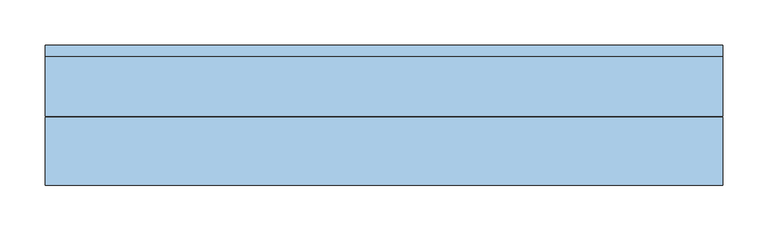
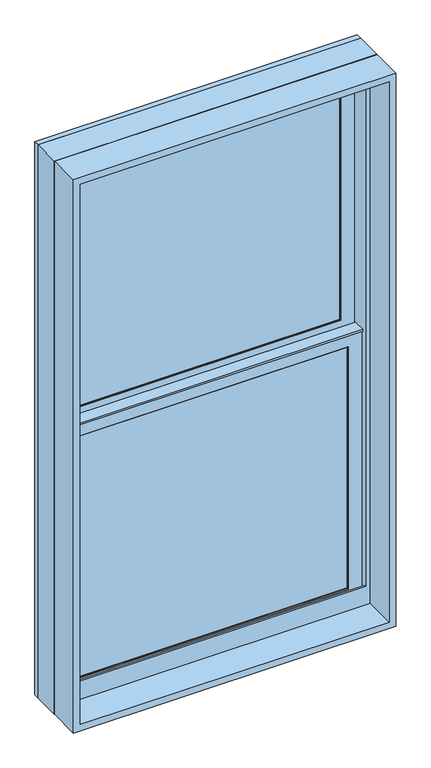
"""IFC4 building model written with IfcOpenShell, lengths in millimetres: window geometry, Window-Double_Hung-Marvin-Essential : ESDH2646."""

from ifc_helpers import new_model, si_unit, frame, origin, place, context, project, spatial, polyline, outline, extrude, faceted_brep, source, transform, mapped, element, save


def window_ea2262a4(model_context):
    return source(origin(), model_context, "Body", "SolidModel", [
        extrude(outline(polyline([(115.3583333, 20.6375), (115.3583333, 15.875), (96.3083333, 15.875), (96.3083333, 20.6375), (115.3583333, 20.6375)])), frame((0.0, 0.0, 1136.65), z_axis=(0.0, 0.0, 1.0), x_axis=(1.0, 0.0, 0.0)), (0.0, 0.0, 1.0), 603.25),
        extrude(outline(polyline([(-96.3083333, 20.6375), (-96.3083333, 15.875), (-115.3583333, 15.875), (-115.3583333, 20.6375), (-96.3083333, 20.6375)])), frame((0.0, 0.0, 1136.65), z_axis=(0.0, 0.0, 1.0), x_axis=(1.0, 0.0, 0.0)), (0.0, 0.0, 1.0), 603.25),
        extrude(outline(polyline([(317.5, 20.6375), (317.5, 15.875), (-317.5, 15.875), (-317.5, 20.6375), (317.5, 20.6375)])), frame((0.0, 0.0, 1428.75), z_axis=(0.0, 0.0, 1.0), x_axis=(1.0, 0.0, 0.0)), (0.0, 0.0, 1.0), 19.05),
        extrude(outline(polyline([(-115.3583333, 46.83125), (-115.3583333, 51.59375), (-96.3083333, 51.59375), (-96.3083333, 46.83125), (-115.3583333, 46.83125)])), frame((0.0, 0.0, 1778.0), z_axis=(0.0, 0.0, 1.0), x_axis=(1.0, 0.0, 0.0)), (0.0, 0.0, 1.0), 603.25),
        extrude(outline(polyline([(96.3083333, 46.83125), (96.3083333, 51.59375), (115.3583333, 51.59375), (115.3583333, 46.83125), (96.3083333, 46.83125)])), frame((0.0, 0.0, 1778.0), z_axis=(0.0, 0.0, 1.0), x_axis=(1.0, 0.0, 0.0)), (0.0, 0.0, 1.0), 603.25),
        extrude(outline(polyline([(-317.5, 46.83125), (-317.5, 51.59375), (317.5, 51.59375), (317.5, 46.83125), (-317.5, 46.83125)])), frame((0.0, 0.0, 2070.1), z_axis=(0.0, 0.0, 1.0), x_axis=(1.0, 0.0, 0.0)), (0.0, 0.0, 1.0), 19.05),
        extrude(outline(polyline([(115.3583333, 20.6375), (96.3083333, 20.6375), (96.3083333, 25.4), (115.3583333, 25.4), (115.3583333, 20.6375)])), frame((0.0, 0.0, 1136.65), z_axis=(0.0, 0.0, 1.0), x_axis=(1.0, 0.0, 0.0)), (0.0, 0.0, 1.0), 603.25),
        extrude(outline(polyline([(-96.3083333, 20.6375), (-115.3583333, 20.6375), (-115.3583333, 25.4), (-96.3083333, 25.4), (-96.3083333, 20.6375)])), frame((0.0, 0.0, 1136.65), z_axis=(0.0, 0.0, 1.0), x_axis=(1.0, 0.0, 0.0)), (0.0, 0.0, 1.0), 603.25),
        extrude(outline(polyline([(317.5, 20.6375), (-317.5, 20.6375), (-317.5, 25.4), (317.5, 25.4), (317.5, 20.6375)])), frame((0.0, 0.0, 1428.75), z_axis=(0.0, 0.0, 1.0), x_axis=(1.0, 0.0, 0.0)), (0.0, 0.0, 1.0), 19.05),
        extrude(outline(polyline([(-115.3583333, 56.35625), (-96.3083333, 56.35625), (-96.3083333, 51.59375), (-115.3583333, 51.59375), (-115.3583333, 56.35625)])), frame((0.0, 0.0, 1778.0), z_axis=(0.0, 0.0, 1.0), x_axis=(1.0, 0.0, 0.0)), (0.0, 0.0, 1.0), 603.25),
        extrude(outline(polyline([(96.3083333, 56.35625), (115.3583333, 56.35625), (115.3583333, 51.59375), (96.3083333, 51.59375), (96.3083333, 56.35625)])), frame((0.0, 0.0, 1778.0), z_axis=(0.0, 0.0, 1.0), x_axis=(1.0, 0.0, 0.0)), (0.0, 0.0, 1.0), 603.25),
        extrude(outline(polyline([(-317.5, 56.35625), (317.5, 56.35625), (317.5, 51.59375), (-317.5, 51.59375), (-317.5, 56.35625)])), frame((0.0, 0.0, 2070.1), z_axis=(0.0, 0.0, 1.0), x_axis=(1.0, 0.0, 0.0)), (0.0, 0.0, 1.0), 19.05),
        faceted_brep([(-344.4875, 5.6780605, 1769.9351748), (-344.4875, 5.6780605, 1765.3), (344.4875, 5.6780605, 1765.3), (344.4875, 5.6780605, 1769.9351748), (-344.4875, 34.8118605, 1769.9351748), (344.4875, 34.8118605, 1769.9351748), (344.4875, 34.8118605, 1765.3), (-344.4875, 34.8118605, 1765.3), (-344.4875, 30.1625, 1765.3), (-344.4875, 30.1625, 1109.6625), (-344.4875, 8.9241104, 1109.6625), (-344.4875, 8.9241104, 1765.3), (344.4875, 8.9241104, 1765.3), (344.4875, 30.1625, 1765.3), (344.4875, 8.9241104, 1109.6625), (344.4875, 30.1625, 1109.6625), (-328.6034752, 11.90625, 1751.0034752), (-328.6034752, 30.1625, 1751.0034752), (328.6034752, 30.1625, 1751.0034752), (328.6034752, 11.90625, 1751.0034752), (-311.94375, 10.4662439, 1734.34375), (-311.94375, 11.90625, 1734.34375), (311.94375, 11.90625, 1734.34375), (311.94375, 10.4662439, 1734.34375), (313.4858834, 8.9241104, 1735.8858834), (-313.4858834, 8.9241104, 1735.8858834), (328.6034752, 30.1625, 1125.5465248), (328.6034752, 11.90625, 1125.5465248), (311.94375, 11.90625, 1142.20625), (311.94375, 10.4662439, 1142.20625), (313.4858834, 8.9241104, 1140.6641166), (-328.6034752, 30.1625, 1125.5465248), (-328.6034752, 11.90625, 1125.5465248), (-311.94375, 11.90625, 1142.20625), (-311.94375, 10.4662439, 1142.20625), (-313.4858834, 8.9241104, 1140.6641166)], [[[0, 1, 2, 3]], [[4, 5, 6, 7]], [[1, 0, 4, 7, 8, 9, 10, 11]], [[2, 1, 11, 12]], [[7, 6, 13, 8]], [[3, 2, 12, 14, 15, 13, 6, 5]], [[0, 3, 5, 4]], [[16, 17, 18, 19]], [[20, 21, 22, 23]], [[20, 23, 24, 25]], [[19, 18, 26, 27]], [[23, 22, 28, 29]], [[24, 23, 29, 30]], [[27, 26, 31, 32]], [[29, 28, 33, 34]], [[30, 29, 34, 35]], [[15, 14, 10, 9]], [[15, 9, 8, 13], [18, 17, 31, 26]], [[17, 16, 32, 31]], [[16, 19, 27, 32], [22, 21, 33, 28]], [[21, 20, 34, 33]], [[20, 25, 35, 34]], [[10, 14, 12, 11], [25, 24, 30, 35]]]),
        extrude(outline(polyline([(38.5955581, 1751.0125), (33.5778968, 1751.0125), (33.5778968, 1752.6), (39.9405976, 1752.6), (39.9405976, 1751.0125), (61.515625, 1751.0125), (47.6307501, 1747.6975159), (38.5955581, 1747.6975159), (38.5955581, 1751.0125)])), frame((-344.4875, 0.0, 0.0), z_axis=(1.0, 0.0, 0.0), x_axis=(0.0, 1.0, 0.0)), (0.0, 0.0, 1.0), 688.975),
        faceted_brep([(374.65, 0.0, 1079.5), (374.65, 0.0, 2438.4), (-374.65, 0.0, 2438.4), (-374.65, 0.0, 1079.5), (348.45625, 0.0, 1140.61875), (-348.45625, 0.0, 1140.61875), (-348.45625, 0.0, 2412.20625), (348.45625, 0.0, 2412.20625), (348.45625, 3.96875, 1079.5), (-348.45625, 3.96875, 1079.5), (-348.45625, 3.96875, 1140.61875), (348.45625, 3.96875, 1140.61875), (-374.65, 65.6828125, 1079.5), (-348.45625, 65.6828125, 1079.5), (348.45625, 65.6828125, 1079.5), (374.65, 65.6828125, 1079.5), (-374.65, 65.6828125, 2438.4), (374.65, 65.6828125, 2438.4), (348.45625, 65.6828125, 2412.20625), (-348.45625, 65.6828125, 2412.20625)], [[[0, 1, 2, 3], [4, 5, 6, 7]], [[8, 9, 10, 11]], [[5, 4, 11, 10]], [[0, 3, 12, 13, 9, 8, 14, 15]], [[13, 12, 16, 17, 15, 14, 18, 19]], [[13, 19, 6, 5, 10, 9]], [[7, 6, 19, 18]], [[18, 14, 8, 11, 4, 7]], [[1, 0, 15, 17]], [[2, 1, 17, 16]], [[3, 2, 16, 12]]]),
        faceted_brep([(348.45625, 30.1625, 1758.95), (346.86875, 30.1625, 1758.95), (346.86875, 30.1625, 1103.8544613), (348.45625, 30.1625, 1103.8544613), (-346.86875, 30.1625, 1758.95), (-348.45625, 30.1625, 1758.95), (-348.45625, 30.1625, 1103.8544613), (-346.86875, 30.1625, 1103.8544613), (346.86875, 63.5, 1758.95), (348.45625, 63.5, 1758.95), (348.45625, 63.5, 1097.3743077), (346.86875, 63.5, 1097.3743077), (-348.45625, 63.5, 1758.95), (-346.86875, 63.5, 1758.95), (-346.86875, 63.5, 1097.3743077), (-348.45625, 63.5, 1097.3743077), (359.7108932, 3.96875, 1108.9460105), (359.7108932, 3.96875, 1079.5), (359.7108932, 65.6828125, 1079.5), (359.7108932, 65.6828125, 1096.950012), (-359.7108932, 3.96875, 1079.5), (-359.7108932, 3.96875, 1108.9460105), (-359.7108932, 65.6828125, 1096.950012), (-359.7108932, 65.6828125, 1079.5), (359.7108932, 78.58125, 1094.4428097), (-359.7108932, 78.58125, 1094.4428097), (-357.6971252, 68.2348864, 1096.4539391), (-339.73135, 68.2348864, 1096.4539391), (-339.73135, 65.6828125, 1096.950012), (339.73135, 65.6828125, 1096.950012), (339.73135, 68.2348864, 1096.4539391), (357.6971252, 68.2348864, 1096.4539391), (-374.65, 65.6828125, 1079.5), (-374.65, 78.5948249, 1079.5), (374.65, 78.5948249, 1079.5), (374.65, 65.6828125, 1079.5), (-374.65, 78.58125, 2438.4), (374.65, 78.58125, 2438.4), (359.7108932, 78.58125, 2423.4608932), (-359.7108932, 78.58125, 2423.4608932), (-374.65, 65.6828125, 2438.4), (-357.6971252, 68.2348864, 2421.4471252), (357.6971252, 68.2348864, 2421.4471252), (339.73135, 68.2348864, 2403.48135), (-339.73135, 68.2348864, 2403.48135), (-339.73135, 65.6828125, 2403.48135), (339.73135, 65.6828125, 2403.48135), (374.65, 65.6828125, 2438.4)], [[[0, 1, 2, 3]], [[4, 5, 6, 7]], [[8, 9, 10, 11]], [[12, 13, 14, 15]], [[1, 8, 11, 2]], [[9, 0, 3, 10]], [[1, 0, 9, 8]], [[5, 4, 13, 12]], [[5, 12, 15, 6]], [[13, 4, 7, 14]], [[16, 17, 18, 19]], [[20, 21, 22, 23]], [[24, 25, 26, 27, 28, 22, 21, 16, 19, 29, 30, 31], [3, 2, 11, 10], [7, 6, 15, 14]], [[17, 16, 21, 20]], [[17, 20, 23, 32, 33, 34, 35, 18]], [[34, 33, 36, 37], [25, 24, 38, 39]], [[33, 32, 40, 36]], [[39, 41, 26, 25]], [[41, 42, 31, 30, 43, 44, 27, 26]], [[44, 45, 28, 27]], [[40, 32, 23, 22, 28, 45, 46, 29, 19, 18, 35, 47]], [[36, 40, 47, 37]], [[39, 38, 42, 41]], [[44, 43, 46, 45]], [[34, 37, 47, 35]], [[42, 38, 24, 31]], [[46, 43, 30, 29]]]),
        extrude(outline(polyline([(324.64375, 11.90625), (-324.64375, 11.90625), (-324.64375, 15.08125), (324.64375, 15.08125), (324.64375, 11.90625)])), frame((0.0, 0.0, 1129.50625), z_axis=(0.0, 0.0, 1.0), x_axis=(1.0, 0.0, 0.0)), (0.0, 0.0, 1.0), 617.5375),
        extrude(outline(polyline([(324.64375, 42.8625), (-324.64375, 42.8625), (-324.64375, 46.0375), (324.64375, 46.0375), (324.64375, 42.8625)])), frame((0.0, 0.0, 1770.85625), z_axis=(0.0, 0.0, 1.0), x_axis=(1.0, 0.0, 0.0)), (0.0, 0.0, 1.0), 617.5375),
        faceted_brep([(-311.94375, 31.194477, 1734.34375), (-313.4858834, 32.7366104, 1735.8858834), (313.4858834, 32.7366104, 1735.8858834), (311.94375, 31.194477, 1734.34375), (-311.94375, 30.1625, 1734.34375), (311.94375, 30.1625, 1734.34375), (-344.4875, 32.7366104, 1766.8875), (-344.4875, 30.1625, 1766.8875), (344.4875, 30.1625, 1766.8875), (344.4875, 32.7366104, 1766.8875), (313.4858834, 32.7366104, 1140.6641166), (311.94375, 31.194477, 1142.20625), (311.94375, 30.1625, 1142.20625), (344.4875, 30.1625, 1109.6625), (344.4875, 32.7366104, 1109.6625), (-313.4858834, 32.7366104, 1140.6641166), (-311.94375, 31.194477, 1142.20625), (-311.94375, 30.1625, 1142.20625), (-344.4875, 30.1625, 1109.6625), (-344.4875, 32.7366104, 1109.6625)], [[[0, 1, 2, 3]], [[4, 0, 3, 5]], [[6, 7, 8, 9]], [[3, 2, 10, 11]], [[5, 3, 11, 12]], [[9, 8, 13, 14]], [[11, 10, 15, 16]], [[12, 11, 16, 17]], [[14, 13, 18, 19]], [[9, 14, 19, 6], [1, 15, 10, 2]], [[16, 15, 1, 0]], [[17, 16, 0, 4]], [[7, 18, 13, 8], [5, 12, 17, 4]], [[19, 18, 7, 6]]]),
        faceted_brep([(-328.6034752, 42.8625, 2392.3534752), (-328.6034752, 61.11875, 2392.3534752), (328.6034752, 61.11875, 2392.3534752), (328.6034752, 42.8625, 2392.3534752), (-311.94375, 41.4224939, 2375.69375), (-311.94375, 42.8625, 2375.69375), (311.94375, 42.8625, 2375.69375), (311.94375, 41.4224939, 2375.69375), (-313.4858834, 39.8803604, 2377.2358834), (313.4858834, 39.8803604, 2377.2358834), (-344.4875, 61.11875, 2408.2375), (-344.4875, 39.8803604, 2408.2375), (344.4875, 39.8803604, 2408.2375), (344.4875, 61.11875, 2408.2375), (328.6034752, 61.11875, 1766.8965248), (328.6034752, 42.8625, 1766.8965248), (311.94375, 42.8625, 1783.55625), (311.94375, 41.4224939, 1783.55625), (313.4858834, 39.8803604, 1782.0141166), (344.4875, 39.8803604, 1751.0125), (344.4875, 61.11875, 1751.0125), (-328.6034752, 61.11875, 1766.8965248), (-328.6034752, 42.8625, 1766.8965248), (-311.94375, 42.8625, 1783.55625), (-311.94375, 41.4224939, 1783.55625), (-313.4858834, 39.8803604, 1782.0141166), (-344.4875, 39.8803604, 1751.0125), (-344.4875, 61.11875, 1751.0125)], [[[0, 1, 2, 3]], [[4, 5, 6, 7]], [[8, 4, 7, 9]], [[10, 11, 12, 13]], [[3, 2, 14, 15]], [[7, 6, 16, 17]], [[9, 7, 17, 18]], [[13, 12, 19, 20]], [[15, 14, 21, 22]], [[17, 16, 23, 24]], [[18, 17, 24, 25]], [[20, 19, 26, 27]], [[13, 20, 27, 10], [1, 21, 14, 2]], [[22, 21, 1, 0]], [[3, 15, 22, 0], [5, 23, 16, 6]], [[24, 23, 5, 4]], [[25, 24, 4, 8]], [[11, 26, 19, 12], [9, 18, 25, 8]], [[27, 26, 11, 10]]]),
        faceted_brep([(-344.4875, 61.11875, 1751.0125), (-344.4875, 63.6928604, 1751.0125), (344.4875, 63.6928604, 1751.0125), (344.4875, 61.11875, 1751.0125), (-311.94375, 62.150727, 1783.55625), (-311.94375, 61.11875, 1783.55625), (311.94375, 61.11875, 1783.55625), (311.94375, 62.150727, 1783.55625), (-313.4858834, 63.6928604, 1782.0141166), (313.4858834, 63.6928604, 1782.0141166), (344.4875, 63.6928604, 2408.2375), (344.4875, 61.11875, 2408.2375), (311.94375, 61.11875, 2375.69375), (311.94375, 62.150727, 2375.69375), (313.4858834, 63.6928604, 2377.2358834), (-344.4875, 63.6928604, 2408.2375), (-344.4875, 61.11875, 2408.2375), (-311.94375, 61.11875, 2375.69375), (-311.94375, 62.150727, 2375.69375), (-313.4858834, 63.6928604, 2377.2358834)], [[[0, 1, 2, 3]], [[4, 5, 6, 7]], [[8, 4, 7, 9]], [[3, 2, 10, 11]], [[7, 6, 12, 13]], [[9, 7, 13, 14]], [[11, 10, 15, 16]], [[13, 12, 17, 18]], [[14, 13, 18, 19]], [[16, 15, 1, 0]], [[3, 11, 16, 0], [5, 17, 12, 6]], [[18, 17, 5, 4]], [[19, 18, 4, 8]], [[1, 15, 10, 2], [9, 14, 19, 8]]]),
        extrude(outline(polyline([(324.64375, 26.19375), (-324.64375, 26.19375), (-324.64375, 30.1625), (324.64375, 30.1625), (324.64375, 26.19375)])), frame((0.0, 0.0, 1129.50625), z_axis=(0.0, 0.0, 1.0), x_axis=(1.0, 0.0, 0.0)), (0.0, 0.0, 1.0), 617.5375),
        extrude(outline(polyline([(324.64375, 57.15), (-324.64375, 57.15), (-324.64375, 61.11875), (324.64375, 61.11875), (324.64375, 57.15)])), frame((0.0, 0.0, 1770.85625), z_axis=(0.0, 0.0, 1.0), x_axis=(1.0, 0.0, 0.0)), (0.0, 0.0, 1.0), 617.5375),
        extrude(outline(polyline([(2438.4, 374.65), (2438.4, -374.65), (1079.5, -374.65), (1079.5, 374.65), (2438.4, 374.65)]), holes=[polyline([(2422.525, 358.775), (1095.375, 358.775), (1095.375, -358.775), (2422.525, -358.775), (2422.525, 358.775)])]), frame((0.0, -76.2, 0.0), z_axis=(0.0, 1.0, 0.0), x_axis=(0.0, 0.0, 1.0)), (0.0, 0.0, 1.0), 75.40625),
    ])


if __name__ == "__main__":
    model = new_model("IFC4")
    model_context = context("Model", 3, world=origin())
    ifc_project = project(units=[si_unit("LENGTHUNIT", "METRE", prefix="MILLI")], contexts=[model_context])
    site = spatial("IfcSite", under=ifc_project)
    building = spatial("IfcBuilding", under=site)
    placement = place(None, origin())
    window_shape = window_ea2262a4(model_context)
    element("IfcWindow", 1, ObjectType="Window-Double_Hung-Marvin-Essential : ESDH2646", at=placement, inside=building, context=model_context, shape_type="MappedRepresentation", body=[
        mapped(window_shape, transform((0.0, 0.0, 0.0), x_axis=(1.0, 0.0, 0.0), y_axis=(0.0, 1.0, 0.0), z_axis=(0.0, 0.0, 1.0))),
    ])
    save(model, "model.ifc")

# Revit data of these elements
# Type "Window-Double_Hung-Marvin-Essential : ESDH2646"
#   Type Mark = "56"
#   Window Type = "Essential Double Hung"
#   Product data url = "https://bimobject.com/marvin-windows-and-doors/product/marvin-dhwau"
#   Product Guid = "c4a96547-874c-4385-91dc-a058adc19d98"
#   Frame = "All Ultrex"
#   Egress Window = "No"
#   URL = "www.marvin.com"
#   Model = "ESDH2646"
#   Manufacturer = "Marvin Windows and Doors"
#   Label Egress = ""
#   Glass Type = "IG Low E II with Argon"
#   Design Pressure = "DP50"
#   Description = "3054 DBHG"
#   Analytic Construction = "<None>"
#   Prairie Corner Width = 0' - 4"
#   Prairie Corner Height = 0' - 4"
#   Egress Width = 2' - 2 9/16"
#   Egress Height = 1' - 10 27/128"
#   Rough Width = 2' - 6"
#   Rough Height = 4' - 6"
#   Nominal Width = 2' - 6"
#   Nominal Height = 4' - 6"
#   Inset to Installation Flange [instance default] = 0' - 1"
#   Height = 4' - 5 1/2"
#   Egress Area = 4.09707 SF
#   Default Head Height = 8' - 0"
#   Width = 2' - 5 1/2"
#   Daylight Area = 7.95296 SF
#   DLO Width = 2' - 0 9/16"
#   DLO Height = 1' - 11 5/16"
#   Muntins Top Sash = yes
#   Lites Wide Top Sash = 3
#   Lites Wide Bottom Sash = 3
#   Lites High Top Sash = 2
#   Lites High Bottom Sash = 2
#   Lite Cut Prairie 9 = no
#   Lite Cut HV Grid = yes
#   Muntins Bottom Sash = yes
#   Label Visibility = no
#   Jamb Extension Visibility = yes
#   Edition number = 1
#   Interior Material = Ultrex-Marvin-Stonewhite
#   Glazing Material = Glass-Marvin-IG Low E II with Argon
#   Cladding Material = Ultrex-Marvin-Pebblegray
#   Wall Closure = (empty or 0)
#   Assembly Code = ""
# Element 1 (IfcWindow, "Window-Double_Hung-Marvin-Essential : ESDH2646")
#   Materials on its faces: "Ultrex-Marvin-Pebblegray", "Ultrex-Marvin-Stonewhite", "Glass-Marvin-IG Low E II with Argon"
# Materials
#   "Ultrex-Marvin-Stonewhite": class "Paint", colour RGB 250 251 245, transparency 0
#   "Glass-Marvin-IG Low E II with Argon": class "Glass", colour RGB 0 128 192, transparency 0.85
#   "Ultrex-Marvin-Pebblegray": class "Paint", colour RGB 189 185 173, transparency 0
